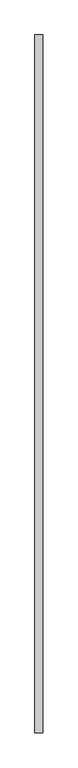
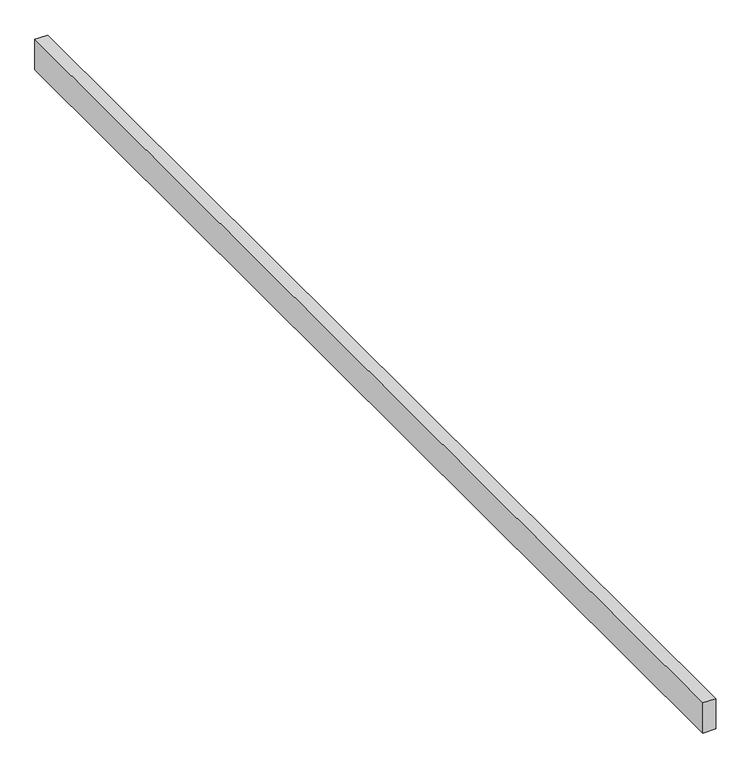
"""IFC4 building model written with IfcOpenShell, lengths in millimetres: proxy geometry, Generic Models 7:Generic Models 1:6:Generic Models 1:6 : Generic Models 7:Generic Models 1:337419:10 : Generic Models 7:Generic Models 1:6:Generic Models 1:6 : Generic Models 7:Generic Models 1:337419:312901."""

from ifc_helpers import new_model, si_unit, frame, origin, place, context, project, spatial, polyline, outline, extrude, source, transform, mapped, element, save


def generic_models_bf65a7a6(model_context):
    return source(origin(), model_context, "Body", "SweptSolid", [
        extrude(outline(polyline([(-70.4425525, 668133.5504931), (-60.1164881, 667637.8994054), (-1293.8930223, 667637.8994054), (-1293.8930223, 668133.5504931), (-70.4425525, 668133.5504931)])), frame((0.0, -578051.3663841, 0.0), z_axis=(0.0, 1.0, 0.0), x_axis=(0.0, 0.0, 1.0)), (0.0, 0.0, 1.0), 44500.8),
    ])


if __name__ == "__main__":
    model = new_model("IFC4")
    model_context = context("Model", 3, world=origin())
    ifc_project = project(units=[si_unit("LENGTHUNIT", "METRE", prefix="MILLI")], contexts=[model_context])
    site = spatial("IfcSite", under=ifc_project)
    building = spatial("IfcBuilding", under=site)
    placement = place(None, origin())
    generic_models_shape = generic_models_bf65a7a6(model_context)
    element("IfcBuildingElementProxy", 1, Name="Generic Models 7:Generic Models 1:6:Generic Models 1:6 : Generic Models 7:Generic Models 1:337419:10 : Generic Models 7:Generic Models 1:6:Generic Models 1:6 : Generic Models 7:Generic Models 1:337419:312901", ObjectType="Generic Models 7:Generic Models 1:6:Generic Models 1:6 : Generic Models 7:Generic Models 1:337419:10 : Generic Models 7:Generic Models 1:6:Generic Models 1:6 : Generic Models 7:Generic Models 1:337419:312901", at=placement, inside=building, context=model_context, shape_type="MappedRepresentation", body=[
        mapped(generic_models_shape, transform((0.0, 0.0, 0.0), x_axis=(1.0, 0.0, 0.0), y_axis=(0.0, 1.0, 0.0), z_axis=(0.0, 0.0, 1.0))),
    ])
    save(model, "model.ifc")

# Revit data of these elements
# Type "Generic Models 7:Generic Models 1:6:Generic Models 1:6 : Generic Models 7:Generic Models 1:337419:10 : Generic Models 7:Generic Models 1:6:Generic Models 1:6 : Generic Models 7:Generic Models 1:337419:312901"
#   NameOverride = "Generic Models 7:Generic Models 1:6:Generic Models 1:6 : Generic Models 7:Generic Models 1:337419:312901"
#   ObjectTypeOverride = "Generic Models 1:6 : Generic Models 7:Generic Models 1:337419"
#   Reference = "Generic Models 1"
#   Tag = "312901"
